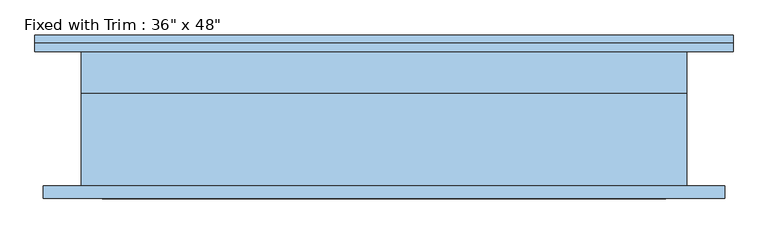
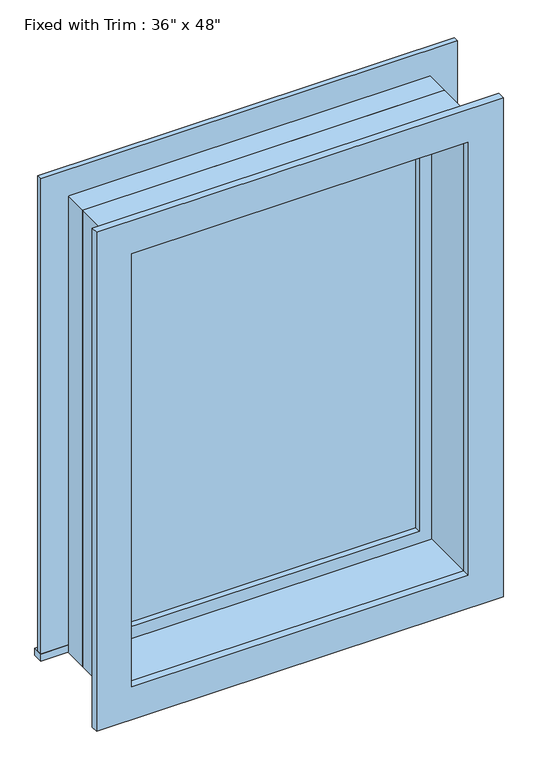
"""IFC4 building model written with IfcOpenShell, lengths in millimetres: window geometry."""

import ifcopenshell
import ifcopenshell.guid

model = None  # the IFC model being written
_history = None  # IfcOwnerHistory: only IFC2X3 demands one
_inside = {}  # id of a spatial element -> (the spatial element, [elements in it])
_under = {}  # id of a project, library or spatial element -> (it, [spatial elements below it])
_declared = {}  # id of a project -> (the project, [libraries it declares])
_typed = {}  # id of a type object -> (the type object, [elements of that type])
_made_of = {}  # id of a material, layer set ... -> (it, [elements and type objects made of it])


def new_model(schema):
    """Start an empty IFC model of exactly this schema.

    Asked for "IFC4X3", IfcOpenShell would pick the latest addendum, in which some entities
    have other attributes; the version numbers below select the first issue.
    IFC2X3 requires an IfcOwnerHistory on every rooted entity: one is made here for all.
    """
    global model, _history
    if schema == "IFC4X3":
        model = ifcopenshell.file(schema_version=(4, 3, 0, 0))
    else:
        model = ifcopenshell.file(schema=schema)
    _inside.clear()
    _under.clear()
    _declared.clear()
    _typed.clear()
    _made_of.clear()
    _history = None
    if model.schema == "IFC2X3":
        org = make("IfcOrganization", Name="unknown")
        user = make(
            "IfcPersonAndOrganization",
            ThePerson=make("IfcPerson", FamilyName="unknown"),
            TheOrganization=org,
        )
        app = make(
            "IfcApplication",
            ApplicationDeveloper=org,
            Version="unknown",
            ApplicationFullName="unknown",
            ApplicationIdentifier="unknown",
        )
        _history = make(
            "IfcOwnerHistory",
            OwningUser=user,
            OwningApplication=app,
            ChangeAction="ADDED",
            CreationDate=0,
        )
    return model


def make(cls, **values):
    """One entity of the class cls with the attributes given. An attribute that is None is left unset."""
    return model.create_entity(
        cls, **{name: value for name, value in values.items() if value is not None}
    )


def rooted(cls, **values):
    """An entity with a GlobalId (a new one), such as an element, a storey or a relation."""
    return make(cls, GlobalId=ifcopenshell.guid.new(), OwnerHistory=_history, **values)


def si_unit(unit_type, name, prefix=None):
    """IfcSIUnit, for example si_unit("LENGTHUNIT", "METRE", prefix="MILLI")."""
    return make("IfcSIUnit", UnitType=unit_type, Prefix=prefix, Name=name)


def assignment(units):
    """IfcUnitAssignment: the units of a project."""
    return None if units is None else make("IfcUnitAssignment", Units=units)


def point(xyz):
    """IfcCartesianPoint."""
    return None if xyz is None else make("IfcCartesianPoint", Coordinates=xyz)


def direction(xyz):
    """IfcDirection."""
    return None if xyz is None else make("IfcDirection", DirectionRatios=xyz)


def frame(location, z_axis=None, x_axis=None):
    """IfcAxis2Placement3D, a coordinate frame: its origin and axes. An axis left out is left unset."""
    return make(
        "IfcAxis2Placement3D",
        Location=point(location),
        Axis=direction(z_axis),
        RefDirection=direction(x_axis),
    )


def origin():
    """The frame at (0, 0, 0) with its axes left unset."""
    return frame((0.0, 0.0, 0.0))


def place(relative_to, where):
    """IfcLocalPlacement: puts the frame where relative to a parent placement (None: the world)."""
    return make(
        "IfcLocalPlacement", PlacementRelTo=relative_to, RelativePlacement=where
    )


def context(
    kind, dimensions, precision=None, world=None, true_north=None, identifier=None
):
    """IfcGeometricRepresentationContext, for example the 3D "Model" context."""
    return make(
        "IfcGeometricRepresentationContext",
        ContextIdentifier=identifier,
        ContextType=kind,
        CoordinateSpaceDimension=dimensions,
        Precision=precision,
        WorldCoordinateSystem=world,
        TrueNorth=true_north,
    )


def project(units=None, contexts=None):
    """IfcProject with its units and contexts."""
    return rooted(
        "IfcProject",
        Name="project",
        RepresentationContexts=contexts,
        UnitsInContext=assignment(units),
    )


def spatial(cls, under=None, at=None, **own):
    """A site, building, storey or space (cls), placed at a placement, below another one or the project."""
    s = rooted(cls, ObjectPlacement=at, **own)
    if under is not None:
        _under.setdefault(under.id(), (under, []))[1].append(s)
    return s


def polyline(points):
    """IfcPolyline through the points."""
    return make("IfcPolyline", Points=[point(p) for p in points])


def outline(outer, holes=None, kind="AREA"):
    """IfcArbitraryClosedProfileDef: a profile drawn as a closed curve; with holes, ...WithVoids."""
    if holes is None:
        return make("IfcArbitraryClosedProfileDef", ProfileType=kind, OuterCurve=outer)
    return make(
        "IfcArbitraryProfileDefWithVoids",
        ProfileType=kind,
        OuterCurve=outer,
        InnerCurves=holes,
    )


def extrude(swept, where, along, depth):
    """IfcExtrudedAreaSolid: the profile swept, set in the frame where, extruded along a direction by depth."""
    return make(
        "IfcExtrudedAreaSolid",
        SweptArea=swept,
        Position=where,
        ExtrudedDirection=direction(along),
        Depth=depth,
    )


def shape(context_of_items, identifier, shape_type, items):
    """IfcShapeRepresentation: the items that make up one representation, for example the "Body"."""
    return make(
        "IfcShapeRepresentation",
        ContextOfItems=context_of_items,
        RepresentationIdentifier=identifier,
        RepresentationType=shape_type,
        Items=items,
    )


def source(mapping_origin, context_of_items, identifier, shape_type, items):
    """IfcRepresentationMap: a shape defined once, which mapped items show again and again."""
    return make(
        "IfcRepresentationMap",
        MappingOrigin=mapping_origin,
        MappedRepresentation=shape(context_of_items, identifier, shape_type, items),
    )


def transform(
    local_origin,
    x_axis=None,
    y_axis=None,
    z_axis=None,
    scale=None,
    scale2=None,
    scale3=None,
    uniform=True,
):
    """IfcCartesianTransformationOperator3D, or its non-uniform kind. x_axis, y_axis, z_axis: its Axis1, 2, 3."""
    if uniform:
        return make(
            "IfcCartesianTransformationOperator3D",
            Axis1=direction(x_axis),
            Axis2=direction(y_axis),
            LocalOrigin=point(local_origin),
            Scale=scale,
            Axis3=direction(z_axis),
        )
    return make(
        "IfcCartesianTransformationOperator3DnonUniform",
        Axis1=direction(x_axis),
        Axis2=direction(y_axis),
        LocalOrigin=point(local_origin),
        Scale=scale,
        Axis3=direction(z_axis),
        Scale2=scale2,
        Scale3=scale3,
    )


def mapped(mapping_source, mapping_target):
    """IfcMappedItem: shows the shape of a source again, moved by a transform."""
    return make(
        "IfcMappedItem", MappingSource=mapping_source, MappingTarget=mapping_target
    )


def made_of(thing, what):
    """Note that an element or type object is made of a material, layer set ...; save() writes the relation."""
    if what is not None:
        _made_of.setdefault(what.id(), (what, []))[1].append(thing)
    return thing


def element(
    cls,
    number,
    at=None,
    inside=None,
    cuts=None,
    type_object=None,
    material=None,
    context=None,
    identifier="Body",
    shape_type=None,
    held_by="IfcProductDefinitionShape",
    body=None,
    shapes=None,
    **own,
):
    """One element of the class cls, such as IfcWall. Its Tag is "e" and its number.

    at: its placement. inside: the storey or other place that contains it. cuts: it is an
    opening in that element (IfcRelVoidsElement). A single representation is given by context,
    identifier, shape_type and body (its items); several are given by shapes. held_by: the class
    of the entity that holds the representations. save() writes the other relations.
    """
    e = rooted(cls, Tag="e%d" % number, ObjectPlacement=at, **own)
    if body is not None:
        shapes = [shape(context, identifier, shape_type, body)]
    if shapes is not None:
        e.Representation = make(held_by, Representations=shapes)
    if inside is not None:
        _inside.setdefault(inside.id(), (inside, []))[1].append(e)
    if cuts is not None:
        rooted(
            "IfcRelVoidsElement", RelatingBuildingElement=cuts, RelatedOpeningElement=e
        )
    if type_object is not None:
        _typed.setdefault(type_object.id(), (type_object, []))[1].append(e)
    return made_of(e, material)


def aggregate(whole, parts):
    """IfcRelAggregates: a whole, such as a stair, and the parts it consists of."""
    return rooted("IfcRelAggregates", RelatingObject=whole, RelatedObjects=parts)


def save(model, path):
    """Write the relations noted so far, then the file.

    IfcRelAggregates (storeys below a building ...), IfcRelContainedInSpatialStructure (elements
    in a storey), IfcRelDefinesByType, IfcRelAssociatesMaterial and IfcRelDeclares: one each for
    every whole, place, type object, material and project.
    """
    for whole, parts in _under.values():
        aggregate(whole, parts)
    for where, things in _inside.values():
        rooted(
            "IfcRelContainedInSpatialStructure",
            RelatedElements=things,
            RelatingStructure=where,
        )
    for kind, things in _typed.values():
        rooted("IfcRelDefinesByType", RelatedObjects=things, RelatingType=kind)
    for what, things in _made_of.values():
        rooted("IfcRelAssociatesMaterial", RelatedObjects=things, RelatingMaterial=what)
    for by, libraries in _declared.values():
        rooted("IfcRelDeclares", RelatingContext=by, RelatedDefinitions=libraries)
    model.write(path)


def window_bec2521a(model_context):
    return source(origin(), model_context, "Body", "SweptSolid", [
        extrude(outline(polyline([(-565.15, 127.0), (488.95, 127.0), (488.95, 101.6), (-565.15, 101.6), (-565.15, 127.0)])), frame((0.0, 0.0, 914.4), z_axis=(0.0, 0.0, 1.0), x_axis=(1.0, 0.0, 0.0)), (0.0, 0.0, 1.0), 19.05),
        extrude(outline(polyline([(2114.55, -476.25), (2114.55, 400.05), (933.45, 400.05), (933.45, 488.95), (2203.45, 488.95), (2203.45, -565.15), (933.45, -565.15), (933.45, -476.25), (2114.55, -476.25)])), frame((0.0, 101.6, 0.0), z_axis=(0.0, 1.0, 0.0), x_axis=(0.0, 0.0, 1.0)), (0.0, 0.0, 1.0), 12.7),
        extrude(outline(polyline([(2190.75, 476.25), (2190.75, -552.45), (857.25, -552.45), (857.25, 476.25), (2190.75, 476.25)]), holes=[polyline([(2101.85, 387.35), (946.15, 387.35), (946.15, -463.55), (2101.85, -463.55), (2101.85, 387.35)])]), frame((0.0, -120.65, 0.0), z_axis=(0.0, 1.0, 0.0), x_axis=(0.0, 0.0, 1.0)), (0.0, 0.0, 1.0), 19.05),
        extrude(outline(polyline([(355.6, 53.975), (-431.8, 53.975), (-431.8, 66.675), (355.6, 66.675), (355.6, 53.975)])), frame((0.0, 0.0, 977.9), z_axis=(0.0, 0.0, 1.0), x_axis=(1.0, 0.0, 0.0)), (0.0, 0.0, 1.0), 1092.2),
        extrude(outline(polyline([(2114.55, -476.25), (933.45, -476.25), (933.45, 400.05), (2114.55, 400.05), (2114.55, -476.25)]), holes=[polyline([(2070.1, -431.8), (2070.1, 355.6), (977.9, 355.6), (977.9, -431.8), (2070.1, -431.8)])]), frame((0.0, 38.1, 0.0), z_axis=(0.0, 1.0, 0.0), x_axis=(0.0, 0.0, 1.0)), (0.0, 0.0, 1.0), 44.45),
        extrude(outline(polyline([(2133.6, -495.3), (914.4, -495.3), (914.4, 419.1), (2133.6, 419.1), (2133.6, -495.3)]), holes=[polyline([(2101.85, -463.55), (2101.85, 387.35), (946.15, 387.35), (946.15, -463.55), (2101.85, -463.55)])]), frame((0.0, -101.6, 0.0), z_axis=(0.0, 1.0, 0.0), x_axis=(0.0, 0.0, 1.0)), (0.0, 0.0, 1.0), 139.7),
        extrude(outline(polyline([(2133.6, 419.1), (2133.6, -495.3), (914.4, -495.3), (914.4, 419.1), (2133.6, 419.1)]), holes=[polyline([(2114.55, 400.05), (933.45, 400.05), (933.45, -476.25), (2114.55, -476.25), (2114.55, 400.05)])]), frame((0.0, 38.1, 0.0), z_axis=(0.0, 1.0, 0.0), x_axis=(0.0, 0.0, 1.0)), (0.0, 0.0, 1.0), 63.5),
    ])


if __name__ == "__main__":
    model = new_model("IFC4")
    model_context = context("Model", 3, world=origin())
    ifc_project = project(units=[si_unit("LENGTHUNIT", "METRE", prefix="MILLI")], contexts=[model_context])
    site = spatial("IfcSite", under=ifc_project)
    building = spatial("IfcBuilding", under=site)
    placement = place(None, origin())
    window_shape = window_bec2521a(model_context)
    element("IfcWindow", 1, ObjectType="Fixed with Trim : 36\" x 48\"", at=placement, inside=building, context=model_context, shape_type="MappedRepresentation", body=[
        mapped(window_shape, transform((0.0, 0.0, 0.0), x_axis=(1.0, 0.0, 0.0), y_axis=(0.0, 1.0, 0.0), z_axis=(0.0, 0.0, 1.0))),
    ])
    save(model, "model.ifc")

# Revit data of these elements
# Type "Fixed with Trim : 36\" x 48\""
#   Type Mark = "46"
#   Assembly Code = "B2020100"
#   Height = 4' - 0"
#   Default Sill Height = 3' - 0"
#   Trim Projection - Ext. = 0' - 0 1/2"
#   Trim Projection - Int. = 0' - 0 3/4"
#   Trim Width - Exterior = 0' - 3 1/2"
#   Trim Width - Interior = 0' - 3 1/2"
#   Width = 3' - 0"
#   Window Inset = 0' - 0 3/4"
#   Define Thermal Properties by = 0
#   Glass Pane Material = Glass
#   Sash Material = Sash
#   Trim Exterior Material = Trim
#   Trim Interior Material = Trim
#   Wall Closure = (empty or 0)
# Element 1 (IfcWindow, "Fixed with Trim : 36\" x 48\"")
#   Materials on its faces: "Sash", "Trim", "Glass"
# Materials
#   "Glass": class "Glass", colour RGB 236 240 239, transparency 0.5, Description = "Soda Lime Glass", Cost = 0
#   "Sash": class "Wood", colour RGB 227 170 128, transparency 0, Cost = 0
#   "Trim": class "Wood", colour RGB 227 170 128, transparency 0, Cost = 0
